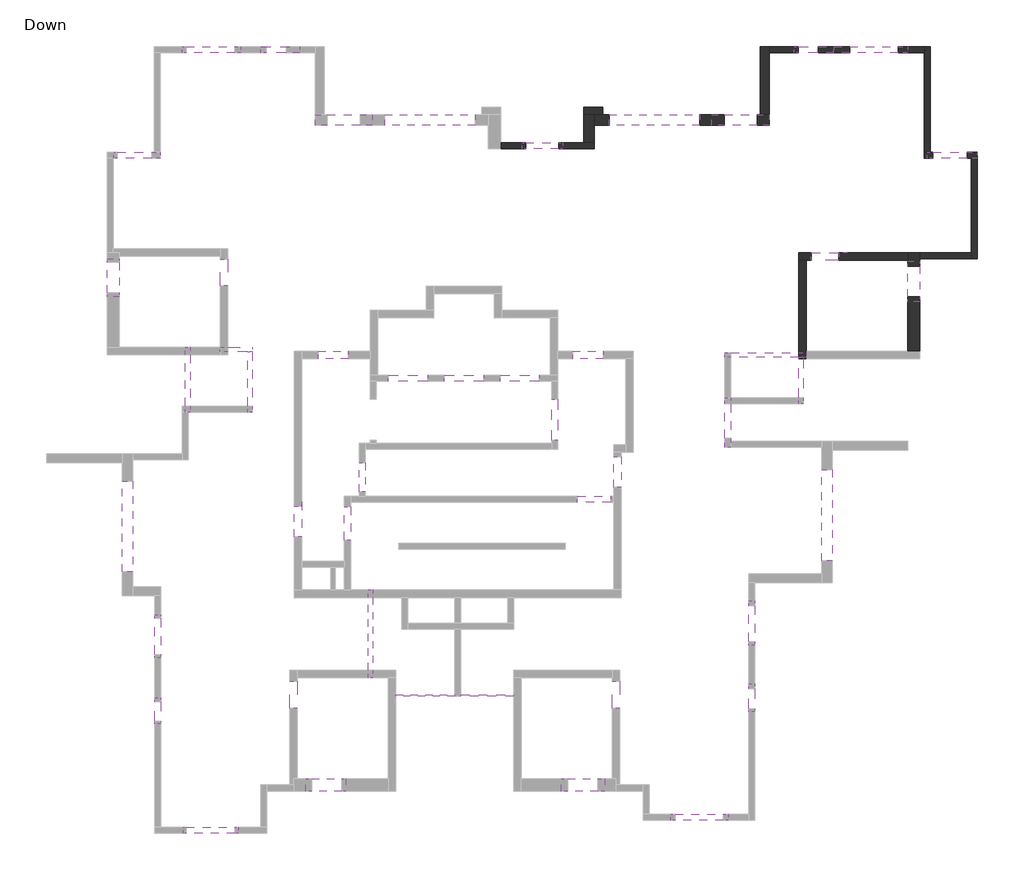
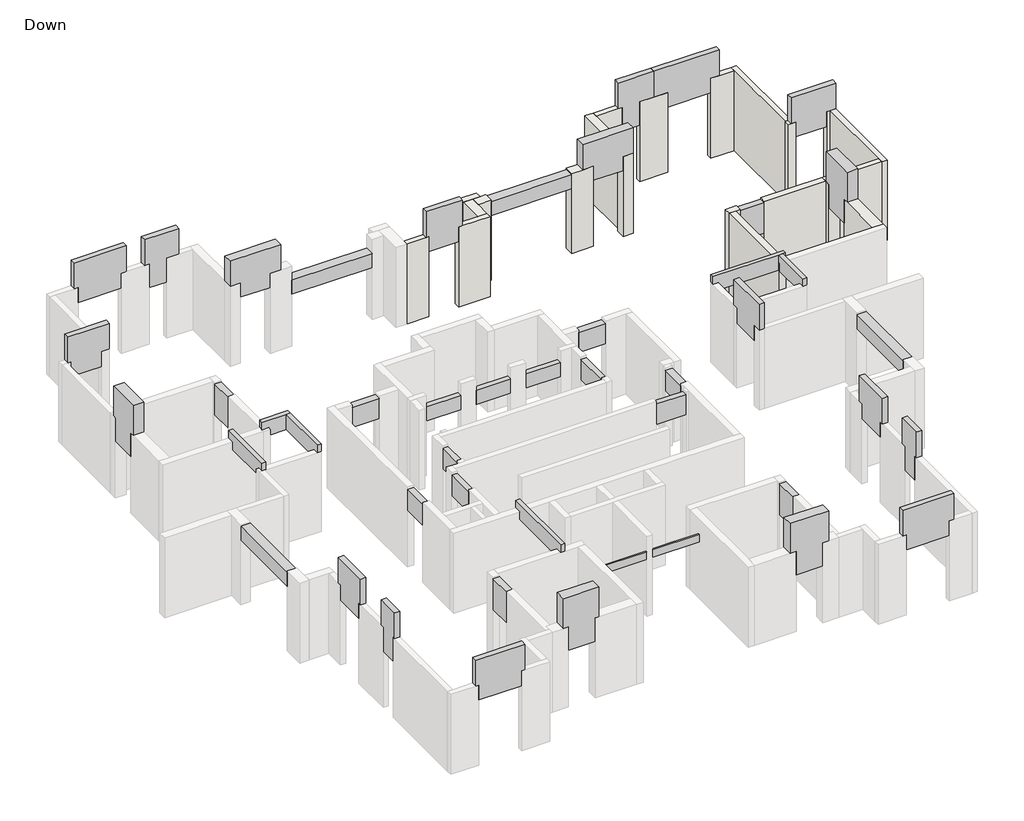
# One storey, part 3 of 3: 47 beams, 21 walls.
# Revit data of these elements (continued)
# Element 15 (IfcBeam, "Concrete Rectengular Beam : 20/160") (continued)
#   SOFiSTiK_AMG_Adjusted = yes
#   Structural Material = Concrete
#   Phase Created = New Construction
#   Materials on its faces: "Concrete"
# Element 16 (IfcBeam, "Concrete Rectengular Beam : 20/160")
#   Comments = ""
#   Mark = "B17"
#   SOFiSTiK_AMG_Comments = ""
#   SOFiSTiK_AMG_Scheduled = yes
#   SOFiSTiK_AMG_Adjusted = yes
#   Structural Material = Concrete
#   Phase Created = New Construction
#   Materials on its faces: "Concrete"
# Element 17 (IfcBeam, "Concrete Rectengular Beam : 20/195")
#   Comments = ""
#   Mark = "B18"
#   SOFiSTiK_AMG_Comments = ""
#   SOFiSTiK_AMG_Scheduled = yes
#   SOFiSTiK_AMG_Adjusted = yes
#   Structural Material = Concrete
#   Phase Created = New Construction
#   Materials on its faces: "Concrete"
# Element 18 (IfcBeam, "Concrete Rectengular Beam : 20/195")
#   Comments = ""
#   Mark = "B19"
#   SOFiSTiK_AMG_Comments = ""
#   SOFiSTiK_AMG_Scheduled = yes
#   SOFiSTiK_AMG_Adjusted = yes
#   Structural Material = Concrete
#   Phase Created = New Construction
#   Materials on its faces: "Concrete"
# Element 19 (IfcBeam, "Concrete Rectengular Beam : 20/195")
#   Comments = ""
#   Mark = "B20"
#   SOFiSTiK_AMG_Comments = ""
#   SOFiSTiK_AMG_Scheduled = yes
#   SOFiSTiK_AMG_Adjusted = yes
#   Structural Material = Concrete
#   Phase Created = New Construction
#   Materials on its faces: "Concrete"
# Element 20 (IfcBeam, "Concrete Rectengular Beam : 20/195")
#   Comments = ""
#   Mark = "B21"
#   SOFiSTiK_AMG_Comments = ""
#   SOFiSTiK_AMG_Scheduled = yes
#   SOFiSTiK_AMG_Adjusted = yes
#   Structural Material = Concrete
#   Phase Created = New Construction
#   Materials on its faces: "Concrete"
# Element 21 (IfcBeam, "Concrete Rectengular Beam : 20/55")
#   Comments = ""
#   Mark = "B22"
#   SOFiSTiK_AMG_Comments = ""
#   SOFiSTiK_AMG_Scheduled = yes
#   SOFiSTiK_AMG_Adjusted = yes
#   Structural Material = Concrete
#   Phase Created = New Construction
#   Materials on its faces: "Concrete"
# Element 22 (IfcBeam, "Concrete Rectengular Beam : 20/55")
#   Comments = ""
#   Mark = "B23"
#   SOFiSTiK_AMG_Comments = ""
#   SOFiSTiK_AMG_Scheduled = yes
#   SOFiSTiK_AMG_Adjusted = yes
#   Structural Material = Concrete
#   Phase Created = New Construction
#   Materials on its faces: "Concrete"
# Element 23 (IfcBeam, "Concrete Rectengular Beam : 20/55")
#   Comments = ""
#   Mark = "B24"
#   SOFiSTiK_AMG_Comments = ""
#   SOFiSTiK_AMG_Scheduled = yes
#   SOFiSTiK_AMG_Adjusted = yes
#   Structural Material = Concrete
#   Phase Created = New Construction
#   Materials on its faces: "Concrete"
# Element 24 (IfcBeam, "Concrete Rectengular Beam : 20/80")
#   Comments = ""
#   Mark = "B25"
#   SOFiSTiK_AMG_Comments = ""
#   SOFiSTiK_AMG_Scheduled = yes
#   SOFiSTiK_AMG_Adjusted = yes
#   Structural Material = Concrete
#   Phase Created = New Construction
#   Materials on its faces: "Concrete"
# Element 25 (IfcBeam, "Concrete Rectengular Beam : 20/80")
#   Comments = ""
#   Mark = "B26"
#   SOFiSTiK_AMG_Comments = ""
#   SOFiSTiK_AMG_Scheduled = yes
#   SOFiSTiK_AMG_Adjusted = yes
#   Structural Material = Concrete
#   Phase Created = New Construction
#   Materials on its faces: "Concrete"
# Element 26 (IfcBeam, "Concrete Rectengular Beam : 20/80")
#   Comments = ""
#   Mark = "B27"
#   SOFiSTiK_AMG_Comments = ""
#   SOFiSTiK_AMG_Scheduled = yes
#   SOFiSTiK_AMG_Adjusted = yes
#   Structural Material = Concrete
#   Phase Created = New Construction
#   Materials on its faces: "Concrete"
# Element 27 (IfcBeam, "Concrete Rectengular Beam : 20/80")
#   Comments = ""
#   Mark = "B28"
#   SOFiSTiK_AMG_Comments = ""
#   SOFiSTiK_AMG_Scheduled = yes
#   SOFiSTiK_AMG_Adjusted = yes
#   Structural Material = Concrete
#   Phase Created = New Construction
#   Materials on its faces: "Concrete"
# Element 28 (IfcBeam, "Concrete Rectengular Beam : 25/120")
#   Comments = ""
#   Mark = "B29"
#   SOFiSTiK_AMG_Comments = ""
#   SOFiSTiK_AMG_Scheduled = yes
#   SOFiSTiK_AMG_Adjusted = yes
#   Structural Material = Concrete
#   Phase Created = New Construction
#   Materials on its faces: "Concrete"
# Element 29 (IfcBeam, "Concrete Rectengular Beam : 25/120")
#   Comments = ""
#   Mark = "B30"
#   SOFiSTiK_AMG_Comments = ""
#   SOFiSTiK_AMG_Scheduled = yes
#   SOFiSTiK_AMG_Adjusted = yes
#   Structural Material = Concrete
#   Phase Created = New Construction
#   Materials on its faces: "Concrete"
# Element 30 (IfcBeam, "Concrete Rectengular Beam : 25/120")
#   Comments = ""
#   Mark = "B31"
#   SOFiSTiK_AMG_Comments = ""
#   SOFiSTiK_AMG_Scheduled = yes
#   SOFiSTiK_AMG_Adjusted = yes
#   Structural Material = Concrete
#   Phase Created = New Construction
#   Materials on its faces: "Concrete"
# Element 31 (IfcBeam, "Concrete Rectengular Beam : 25/120")
#   Comments = ""
#   Mark = "B32"
#   SOFiSTiK_AMG_Comments = ""
#   SOFiSTiK_AMG_Scheduled = yes
#   SOFiSTiK_AMG_Adjusted = yes
#   Structural Material = Concrete
#   Phase Created = New Construction
#   Materials on its faces: "Concrete"
# Element 32 (IfcBeam, "Concrete Rectengular Beam : 25/80")
#   Comments = ""
#   Mark = "B34"
#   SOFiSTiK_AMG_Comments = ""
#   SOFiSTiK_AMG_Scheduled = yes
#   SOFiSTiK_AMG_Adjusted = yes
#   Structural Material = Concrete
#   Phase Created = New Construction
#   Materials on its faces: "Concrete"
# Element 33 (IfcBeam, "Concrete Rectengular Beam : 25/80")
#   Comments = ""
#   Mark = "B35"
#   SOFiSTiK_AMG_Comments = ""
#   SOFiSTiK_AMG_Scheduled = yes
#   SOFiSTiK_AMG_Adjusted = yes
#   Structural Material = Concrete
#   Phase Created = New Construction
#   Materials on its faces: "Concrete"
# Element 34 (IfcBeam, "Concrete Rectengular Beam : 25/80")
#   Comments = ""
#   Mark = "B36"
#   SOFiSTiK_AMG_Comments = ""
#   SOFiSTiK_AMG_Scheduled = yes
#   SOFiSTiK_AMG_Adjusted = yes
#   Structural Material = Concrete
#   Phase Created = New Construction
#   Materials on its faces: "Concrete"
# Element 35 (IfcBeam, "Concrete Rectengular Beam : 25/80")
#   Comments = ""
#   Mark = "B37"
#   SOFiSTiK_AMG_Comments = ""
#   SOFiSTiK_AMG_Scheduled = yes
#   SOFiSTiK_AMG_Adjusted = yes
#   Structural Material = Concrete
#   Phase Created = New Construction
#   Materials on its faces: "Concrete"
# Element 36 (IfcBeam, "Concrete Rectengular Beam : 35/155")
#   Comments = ""
#   Mark = "B38"
#   SOFiSTiK_AMG_Comments = ""
#   SOFiSTiK_AMG_Scheduled = yes
#   SOFiSTiK_AMG_Adjusted = yes
#   Structural Material = Concrete
#   Phase Created = New Construction
#   Materials on its faces: "Concrete"
# Element 37 (IfcBeam, "Concrete Rectengular Beam : 35/155")
#   Comments = ""
#   Mark = "B39"
#   SOFiSTiK_AMG_Comments = ""
#   SOFiSTiK_AMG_Scheduled = yes
#   SOFiSTiK_AMG_Adjusted = yes
#   Structural Material = Concrete
#   Phase Created = New Construction
#   Materials on its faces: "Concrete"
# Element 38 (IfcBeam, "Concrete Rectengular Beam : 35/50")
#   Comments = ""
#   Mark = "B40"
#   SOFiSTiK_AMG_Comments = ""
#   SOFiSTiK_AMG_Scheduled = yes
#   SOFiSTiK_AMG_Adjusted = yes
#   Structural Material = Concrete
#   Phase Created = New Construction
#   Materials on its faces: "Concrete"
# Element 39 (IfcBeam, "Concrete Rectengular Beam : 35/50")
#   Comments = ""
#   Mark = "B41"
#   SOFiSTiK_AMG_Comments = ""
#   SOFiSTiK_AMG_Scheduled = yes
#   SOFiSTiK_AMG_Adjusted = yes
#   Structural Material = Concrete
#   Phase Created = New Construction
#   Materials on its faces: "Concrete"
# Element 40 (IfcBeam, "Concrete Rectengular Beam : 35/50")
#   Comments = ""
#   Mark = "B42"
#   SOFiSTiK_AMG_Comments = ""
#   SOFiSTiK_AMG_Scheduled = yes
#   SOFiSTiK_AMG_Adjusted = yes
#   Structural Material = Concrete
#   Phase Created = New Construction
#   Materials on its faces: "Concrete"
# Element 41 (IfcBeam, "Concrete Rectengular Beam : 35/55")
#   Comments = ""
#   Mark = "B43"
#   SOFiSTiK_AMG_Comments = ""
#   SOFiSTiK_AMG_Scheduled = yes
#   SOFiSTiK_AMG_Adjusted = yes
#   Structural Material = Concrete
#   Phase Created = New Construction
#   Materials on its faces: "Concrete"
# Element 42 (IfcBeam, "Concrete Rectengular Beam : 40/210")
#   Comments = ""
#   Mark = "B44"
#   SOFiSTiK_AMG_Comments = ""
#   SOFiSTiK_AMG_Scheduled = yes
#   SOFiSTiK_AMG_Adjusted = yes
#   Structural Material = Concrete
#   Phase Created = New Construction
#   Materials on its faces: "Concrete"
# Element 43 (IfcBeam, "Concrete Rectengular Beam : 40/210")
#   Comments = ""
#   Mark = "B45"
#   SOFiSTiK_AMG_Comments = ""
#   SOFiSTiK_AMG_Scheduled = yes
#   SOFiSTiK_AMG_Adjusted = yes
#   Structural Material = Concrete
#   Phase Created = New Construction
#   Materials on its faces: "Concrete"
# Element 44 (IfcBeam, "Concrete Rectengular Beam : 40/210")
#   Comments = ""
#   Mark = "B46"
#   SOFiSTiK_AMG_Comments = ""
#   SOFiSTiK_AMG_Scheduled = yes
#   SOFiSTiK_AMG_Adjusted = yes
#   Structural Material = Concrete
#   Phase Created = New Construction
#   Materials on its faces: "Concrete"
# Element 45 (IfcBeam, "Concrete Rectengular Beam : 40/210")
#   Comments = ""
#   Mark = "B47"
#   SOFiSTiK_AMG_Comments = ""
#   SOFiSTiK_AMG_Scheduled = yes
#   SOFiSTiK_AMG_Adjusted = yes
#   Structural Material = Concrete
#   Phase Created = New Construction
#   Materials on its faces: "Concrete"
# Element 46 (IfcBeam, "Concrete Rectengular Beam : 5/30")
#   Comments = ""
#   Mark = "B48"
#   SOFiSTiK_AMG_Comments = "Too Narrow Beam /"
#   SOFiSTiK_AMG_Scheduled = yes
#   SOFiSTiK_AMG_Adjusted = yes
#   Structural Material = Concrete
#   Phase Created = New Construction
#   Materials on its faces: "Concrete"
# Element 47 (IfcBeam, "Concrete Rectengular Beam : 5/30")
#   Comments = ""
#   Mark = "B49"
#   SOFiSTiK_AMG_Comments = "Too Narrow Beam /"
#   SOFiSTiK_AMG_Scheduled = yes
#   SOFiSTiK_AMG_Adjusted = yes
#   Structural Material = Concrete
#   Phase Created = New Construction
#   Materials on its faces: "Concrete"
# Element 48 (IfcWall, "20")
#   Comments = ""
#   Mark = "W14"
#   SOFiSTiK_EdgeZones = "W14"
#   SOFiSTiK_AMG_Comments = ""
#   Top Offset = 0 cm
#   Base Offset = 0 cm
#   wall height = 315 cm
#   SOFiSTiK_AMG_Scheduled = yes
#   SOFiSTiK_AMG_Adjusted = yes
#   Phase Created = New Construction
#   Base Constraint = Down
#   Top Constraint = Typical Floor
#   Materials on its faces: "Concrete"
# Element 49 (IfcWall, "20")
#   Comments = ""
#   Mark = "W19"
#   SOFiSTiK_EdgeZones = "W19"
#   SOFiSTiK_AMG_Comments = ""
#   Top Offset = 0 cm
#   Base Offset = 0 cm
#   wall height = 315 cm
#   SOFiSTiK_AMG_Scheduled = yes
#   SOFiSTiK_AMG_Adjusted = yes
#   Phase Created = New Construction
#   Base Constraint = Down
#   Top Constraint = Typical Floor
#   Materials on its faces: "Concrete"
# Element 50 (IfcWall, "20")
#   Comments = ""
#   Mark = "W20"
#   SOFiSTiK_EdgeZones = "W20"
#   SOFiSTiK_AMG_Comments = ""
#   Top Offset = 0 cm
#   Base Offset = 0 cm
#   wall height = 315 cm
#   SOFiSTiK_AMG_Scheduled = yes
#   SOFiSTiK_AMG_Adjusted = yes
#   Phase Created = New Construction
#   Base Constraint = Down
#   Top Constraint = Typical Floor
#   Materials on its faces: "Concrete"
# Element 51 (IfcWall, "20")
#   Comments = ""
#   Mark = "W21"
#   SOFiSTiK_EdgeZones = "W21"
#   SOFiSTiK_AMG_Comments = ""
#   Top Offset = 0 cm
#   Base Offset = 0 cm
#   wall height = 315 cm
#   SOFiSTiK_AMG_Scheduled = yes
#   SOFiSTiK_AMG_Adjusted = yes
#   Phase Created = New Construction
#   Base Constraint = Down
#   Top Constraint = Typical Floor
#   Materials on its faces: "Concrete"
# Element 52 (IfcWall, "20")
#   Comments = ""
#   Mark = "W22"
#   SOFiSTiK_EdgeZones = "W22"
#   SOFiSTiK_AMG_Comments = ""
#   Top Offset = 0 cm
#   Base Offset = 0 cm
#   wall height = 315 cm
#   SOFiSTiK_AMG_Scheduled = yes
#   SOFiSTiK_AMG_Adjusted = yes
#   Phase Created = New Construction
#   Base Constraint = Down
#   Top Constraint = Typical Floor
#   Materials on its faces: "Concrete"
# Element 53 (IfcWall, "20")
#   Comments = ""
#   Mark = "W23"
#   SOFiSTiK_EdgeZones = "W23"
#   SOFiSTiK_AMG_Comments = ""
#   Top Offset = 0 cm
#   Base Offset = 0 cm
#   wall height = 315 cm
#   SOFiSTiK_AMG_Scheduled = yes
#   SOFiSTiK_AMG_Adjusted = yes
#   Phase Created = New Construction
#   Base Constraint = Down
#   Top Constraint = Typical Floor
#   Materials on its faces: "Concrete"
# Element 54 (IfcWall, "20")
#   Comments = ""
#   Mark = "W65"
#   SOFiSTiK_EdgeZones = "W65"
#   SOFiSTiK_AMG_Comments = ""
#   Top Offset = 0 cm
#   Base Offset = 0 cm
#   wall height = 315 cm
#   SOFiSTiK_AMG_Scheduled = yes
#   SOFiSTiK_AMG_Adjusted = yes
#   Phase Created = New Construction
#   Base Constraint = Down
#   Top Constraint = Typical Floor
#   Materials on its faces: "Concrete"
# Element 55 (IfcWall, "20")
#   Comments = ""
#   Mark = "W66"
#   SOFiSTiK_EdgeZones = "W66"
#   SOFiSTiK_AMG_Comments = ""
#   Top Offset = 0 cm
#   Base Offset = 0 cm
#   wall height = 315 cm
#   SOFiSTiK_AMG_Scheduled = yes
#   SOFiSTiK_AMG_Adjusted = yes
#   Phase Created = New Construction
#   Base Constraint = Down
#   Top Constraint = Typical Floor
#   Materials on its faces: "Concrete"
# Element 56 (IfcWall, "20")
#   Comments = ""
#   Mark = "W67"
#   SOFiSTiK_EdgeZones = "W67"
#   SOFiSTiK_AMG_Comments = ""
#   Top Offset = 0 cm
#   Base Offset = 0 cm
#   wall height = 315 cm
#   SOFiSTiK_AMG_Scheduled = yes
#   SOFiSTiK_AMG_Adjusted = yes
#   Phase Created = New Construction
#   Base Constraint = Down
#   Top Constraint = Typical Floor
#   Materials on its faces: "Concrete"
# Element 57 (IfcWall, "20")
#   Comments = ""
#   Mark = "W68"
#   SOFiSTiK_EdgeZones = "W68"
#   SOFiSTiK_AMG_Comments = ""
#   Top Offset = 0 cm
#   Base Offset = 0 cm
#   wall height = 315 cm
#   SOFiSTiK_AMG_Scheduled = yes
#   SOFiSTiK_AMG_Adjusted = yes
#   Phase Created = New Construction
#   Base Constraint = Down
#   Top Constraint = Typical Floor
#   Materials on its faces: "Concrete"
# Element 58 (IfcWall, "25")
#   Comments = ""
#   Mark = "W85"
#   SOFiSTiK_EdgeZones = "W85"
#   SOFiSTiK_AMG_Comments = ""
#   Top Offset = 0 cm
#   Base Offset = 0 cm
#   wall height = 315 cm
#   SOFiSTiK_AMG_Scheduled = yes
#   SOFiSTiK_AMG_Adjusted = yes
#   Phase Created = New Construction
#   Base Constraint = Down
#   Top Constraint = Typical Floor
#   Materials on its faces: "Concrete"
# Element 59 (IfcWall, "25")
#   Comments = ""
#   Mark = "W86"
#   SOFiSTiK_EdgeZones = "W86"
#   SOFiSTiK_AMG_Comments = ""
#   Top Offset = 0 cm
#   Base Offset = 0 cm
#   wall height = 315 cm
#   SOFiSTiK_AMG_Scheduled = yes
#   SOFiSTiK_AMG_Adjusted = yes
#   Phase Created = New Construction
#   Base Constraint = Down
#   Top Constraint = Typical Floor
#   Materials on its faces: "Concrete"
# Element 60 (IfcWall, "25")
#   Comments = ""
#   Mark = "W87"
#   SOFiSTiK_EdgeZones = "W87"
#   SOFiSTiK_AMG_Comments = ""
#   Top Offset = 0 cm
#   Base Offset = 0 cm
#   wall height = 315 cm
#   SOFiSTiK_AMG_Scheduled = yes
#   SOFiSTiK_AMG_Adjusted = yes
#   Phase Created = New Construction
#   Base Constraint = Down
#   Top Constraint = Typical Floor
#   Materials on its faces: "Concrete"
# Element 61 (IfcWall, "25")
#   Comments = ""
#   Mark = "W88"
#   SOFiSTiK_EdgeZones = "W88"
#   SOFiSTiK_AMG_Comments = ""
#   Top Offset = 0 cm
#   Base Offset = 0 cm
#   wall height = 315 cm
#   SOFiSTiK_AMG_Scheduled = yes
#   SOFiSTiK_AMG_Adjusted = yes
#   Phase Created = New Construction
#   Base Constraint = Down
#   Top Constraint = Typical Floor
#   Materials on its faces: "Concrete"
# Element 62 (IfcWall, "30")
#   Comments = ""
#   Mark = "W76"
#   SOFiSTiK_EdgeZones = "W76"
#   SOFiSTiK_AMG_Comments = ""
#   Top Offset = 0 cm
#   Base Offset = 0 cm
#   wall height = 315 cm
#   SOFiSTiK_AMG_Scheduled = yes
#   SOFiSTiK_AMG_Adjusted = yes
#   Phase Created = New Construction
#   Base Constraint = Down
#   Top Constraint = Typical Floor
#   Materials on its faces: "Concrete"
# Element 63 (IfcWall, "35")
#   Comments = ""
#   Mark = "W5"
#   SOFiSTiK_EdgeZones = "W5"
#   SOFiSTiK_AMG_Comments = ""
#   Top Offset = 0 cm
#   Base Offset = 0 cm
#   wall height = 315 cm
#   SOFiSTiK_AMG_Scheduled = yes
#   SOFiSTiK_AMG_Adjusted = yes
#   Phase Created = New Construction
#   Base Constraint = Down
#   Top Constraint = Typical Floor
#   Materials on its faces: "Concrete"
# Element 64 (IfcWall, "35")
#   Comments = ""
#   Mark = "W6"
#   SOFiSTiK_EdgeZones = "W6"
#   SOFiSTiK_AMG_Comments = ""
#   Top Offset = 0 cm
#   Base Offset = 0 cm
#   wall height = 315 cm
#   SOFiSTiK_AMG_Scheduled = yes
#   SOFiSTiK_AMG_Adjusted = yes
#   Phase Created = New Construction
#   Base Constraint = Down
#   Top Constraint = Typical Floor
#   Materials on its faces: "Concrete"
# Element 65 (IfcWall, "35")
#   Comments = ""
#   Mark = "W7"
#   SOFiSTiK_EdgeZones = "W7"
#   SOFiSTiK_AMG_Comments = ""
#   Top Offset = 0 cm
#   Base Offset = 0 cm
#   wall height = 315 cm
#   SOFiSTiK_AMG_Scheduled = yes
#   SOFiSTiK_AMG_Adjusted = yes
#   Phase Created = New Construction
#   Base Constraint = Down
#   Top Constraint = Typical Floor
#   Materials on its faces: "Concrete"
# Element 66 (IfcWall, "35")
#   Comments = ""
#   Mark = "W8"
#   SOFiSTiK_EdgeZones = "W8"
#   SOFiSTiK_AMG_Comments = ""
#   Top Offset = 0 cm
#   Base Offset = 0 cm
#   wall height = 315 cm
#   SOFiSTiK_AMG_Scheduled = yes
#   SOFiSTiK_AMG_Adjusted = yes
#   Phase Created = New Construction
#   Base Constraint = Down
#   Top Constraint = Typical Floor
#   Materials on its faces: "Concrete"
# Element 67 (IfcWall, "40")
#   Comments = ""
#   Mark = "W117"
#   SOFiSTiK_EdgeZones = "W117"
#   SOFiSTiK_AMG_Comments = ""
#   Top Offset = 0 cm
#   Base Offset = 0 cm
#   wall height = 315 cm
#   SOFiSTiK_AMG_Scheduled = yes
#   SOFiSTiK_AMG_Adjusted = yes
#   Phase Created = New Construction
#   Base Constraint = Down
#   Top Constraint = Typical Floor
#   Materials on its faces: "Concrete"
# Element 68 (IfcWall, "40")
#   Comments = ""
#   Mark = "W120"
#   SOFiSTiK_EdgeZones = "W120"
#   SOFiSTiK_AMG_Comments = ""
#   Top Offset = 0 cm
#   Base Offset = 0 cm
#   wall height = 315 cm
#   SOFiSTiK_AMG_Scheduled = yes
#   SOFiSTiK_AMG_Adjusted = yes
#   Phase Created = New Construction
#   Base Constraint = Down
#   Top Constraint = Typical Floor
#   Materials on its faces: "Concrete"
# Materials
#   "Concrete": class "Concrete", colour RGB 192 192 192, transparency 0, Keynote = "01000", Description = "Cast-in-place concrete", Cost = 0
